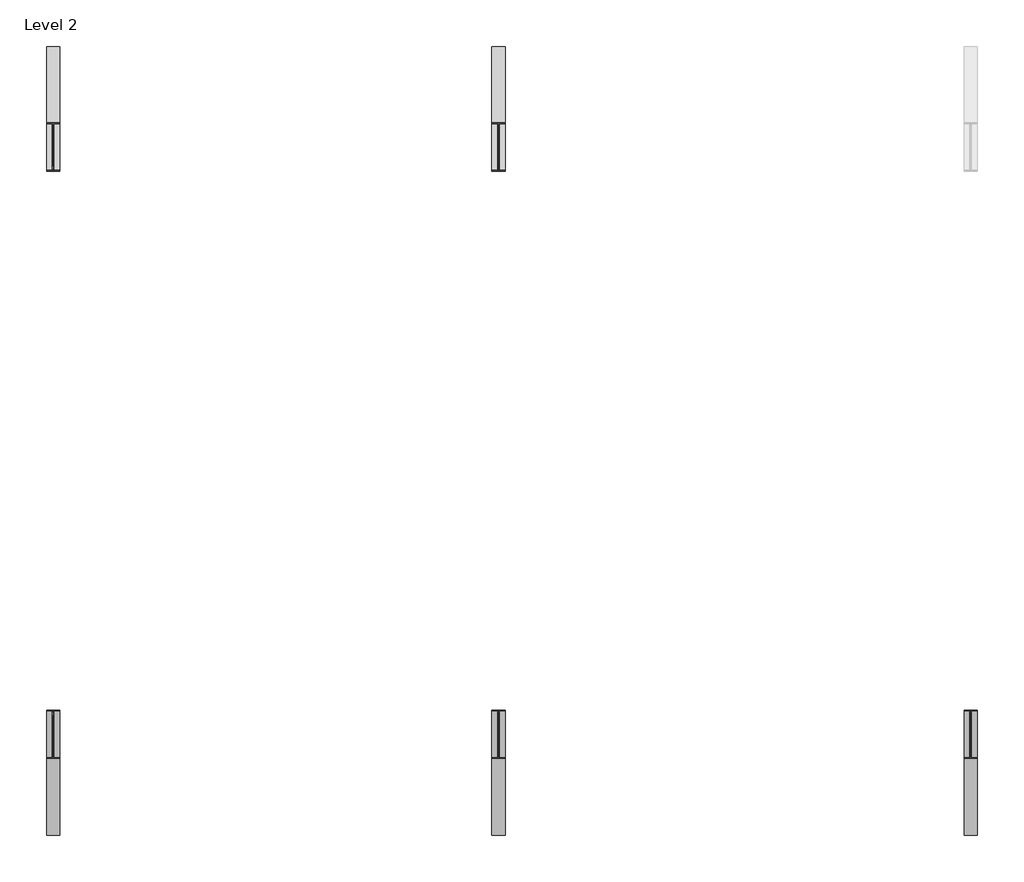
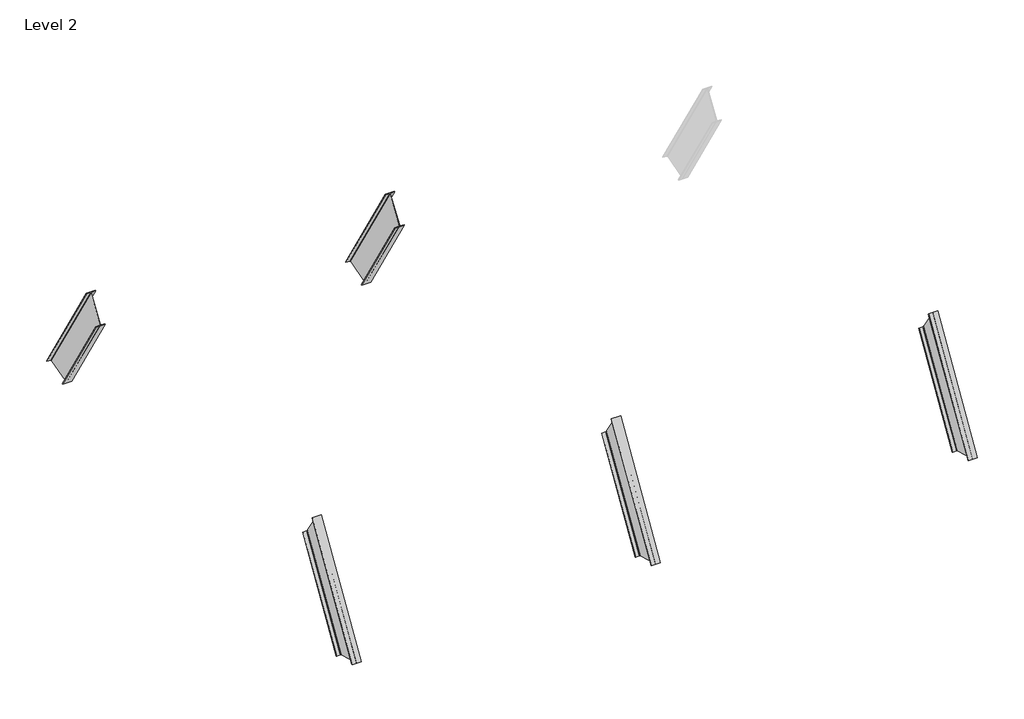
# One storey, part 1 of 2: 5 beams.
"""IFC4 building model written with IfcOpenShell, lengths in millimetres."""

from ifc_helpers import new_model, si_unit, frame, origin, place, context, project, spatial, polyline, ellipse_curve, element, save
from ifc_brep_helpers import plane_surface, revolved_surface, advanced_brep

model = new_model("IFC4")

# Units and contexts
model_context = context("Model", 3, world=origin())
ifc_project = project(units=[si_unit("LENGTHUNIT", "METRE", prefix="MILLI")], contexts=[model_context])

# Site, building, storey
site = spatial("IfcSite", under=ifc_project)
building = spatial("IfcBuilding", under=site)
storey = spatial("IfcBuildingStorey", under=building, Name="Level 2", Elevation=3048.0)

# Beams
placement = place(None, origin())
element("IfcBeam", 1, ObjectType="W Shapes : W 6X18.5", at=placement, inside=storey, context=model_context, shape_type="AdvancedBrep", body=[
    advanced_brep(
    [(18053.8370052, 4087.4629396, 4314.3781499), (17988.1780052, 4087.4629396, 4314.3781499), (17988.1780052, 3103.1094714, 2696.9143292), (18053.8370052, 3103.1094714, 2696.9143292), (17980.5580052, 4082.8387117, 4321.4371423), (17980.5580052, 3095.4894199, 2699.0506628), (17980.5580052, 3818.6411587, 4724.7409096), (17980.5580052, 2660.1304783, 2821.106522), (17988.1780052, 3814.0169308, 4731.799902), (17988.1780052, 2652.5104268, 2823.2428556), (18053.8370052, 3814.0169308, 4731.799902), (18053.8370052, 2652.5104268, 2823.2428556), (18053.8370052, 3808.1595755, 4740.7412924), (18053.8370052, 2642.8583616, 2825.9488782), (17901.4370052, 3808.1595755, 4740.7412924), (17901.4370052, 2642.8583616, 2825.9488782), (17901.4370052, 3814.0169308, 4731.799902), (17901.4370052, 2652.5104268, 2823.2428556), (17967.0960052, 3814.0169308, 4731.799902), (17967.0960052, 2652.5104268, 2823.2428556), (17974.7160052, 3818.6411587, 4724.7409096), (17974.7160052, 2660.1304783, 2821.106522), (17974.7160052, 4082.8387117, 4321.4371423), (17974.7160052, 3095.4894199, 2699.0506628), (17967.0960052, 4087.4629396, 4314.3781499), (17967.0960052, 3103.1094714, 2696.9143292), (17901.4370052, 4087.4629396, 4314.3781499), (17901.4370052, 3103.1094714, 2696.9143292), (17901.4370052, 4093.3202949, 4305.4367595), (17901.4370052, 3112.7615366, 2694.2083066), (18053.8370052, 4093.3202949, 4305.4367595), (18053.8370052, 3112.7615366, 2694.2083066)],
    [
        (0, 1),
        (1, 2),
        (2, 3),
        (3, 0),
        (1, 4, ellipse_curve(frame((17988.1780052, 4082.8387117, 4321.4371423), z_axis=(0.0, 0.8364953080573764, 0.5479740866117624), x_axis=(0.0, 0.5479740866117631, -0.8364953080573758)), 8.4387711, 7.62)),
        (4, 5),
        (5, 2, ellipse_curve(frame((17988.1780052, 3095.4894199, 2699.0506628), z_axis=(0.0, -0.26994852802482067, -0.9628747541696338), x_axis=(0.0, -0.9628747541696336, 0.26994852802482094)), 7.9138553, 7.62)),
        (4, 6),
        (6, 7),
        (7, 5),
        (6, 8, ellipse_curve(frame((17988.1780052, 3818.6411587, 4724.7409096), z_axis=(0.0, 0.8364953080573764, 0.5479740866117624), x_axis=(0.0, 0.5479740866117631, -0.8364953080573758)), 8.4387711, 7.62)),
        (8, 9),
        (9, 7, ellipse_curve(frame((17988.1780052, 2660.1304783, 2821.106522), z_axis=(0.0, -0.26994852802482067, -0.9628747541696338), x_axis=(0.0, -0.9628747541696336, 0.26994852802482094)), 7.9138553, 7.62)),
        (8, 10),
        (10, 11),
        (11, 9),
        (10, 12),
        (12, 13),
        (13, 11),
        (12, 14),
        (14, 15),
        (15, 13),
        (14, 16),
        (16, 17),
        (17, 15),
        (16, 18),
        (18, 19),
        (19, 17),
        (18, 20, ellipse_curve(frame((17967.0960052, 3818.6411587, 4724.7409096), z_axis=(0.0, 0.8364953080573764, 0.5479740866117624), x_axis=(0.0, 0.5479740866117631, -0.8364953080573758)), 8.4387711, 7.62)),
        (20, 21),
        (21, 19, ellipse_curve(frame((17967.0960052, 2660.1304783, 2821.106522), z_axis=(0.0, -0.26994852802482067, -0.9628747541696338), x_axis=(0.0, -0.9628747541696336, 0.26994852802482094)), 7.9138553, 7.62)),
        (20, 22),
        (22, 23),
        (23, 21),
        (22, 24, ellipse_curve(frame((17967.0960052, 4082.8387117, 4321.4371423), z_axis=(0.0, 0.8364953080573764, 0.5479740866117624), x_axis=(0.0, 0.5479740866117631, -0.8364953080573758)), 8.4387711, 7.62)),
        (24, 25),
        (25, 23, ellipse_curve(frame((17967.0960052, 3095.4894199, 2699.0506628), z_axis=(0.0, -0.26994852802482067, -0.9628747541696338), x_axis=(0.0, -0.9628747541696336, 0.26994852802482094)), 7.9138553, 7.62)),
        (24, 26),
        (26, 27),
        (27, 25),
        (26, 28),
        (28, 29),
        (29, 27),
        (28, 30),
        (30, 31),
        (31, 29),
        (30, 0),
        (3, 31),
    ],
    [
        plane_surface(frame((18053.8370052, 4201.324019, 4501.4716915), z_axis=(0.0, -0.8542430559708922, 0.5198738321222864), x_axis=(0.0, -0.5198738321222864, -0.8542430559708922))),
        revolved_surface(polyline([(17980.5580052, 3094.3787005304976, 2697.225557775975), (17980.5580052, 4084.7238158871687, 4324.534696138475)]), (17988.1780052, 4194.8146869, 4505.4331301), (0.0, -0.5198738321222864, -0.8542430559708922)),
        plane_surface(frame((17980.5580052, 4194.8146869, 4505.4331301), z_axis=(1.0000000000000002, 0.0, 0.0), x_axis=(0.0, -0.5198738321222864, -0.8542430559708922))),
        revolved_surface(polyline([(17980.5580052, 2659.0197588679885, 2819.2814170104925), (17980.5580052, 3820.5262629103145, 4727.8384634243885)]), (17988.1780052, 3822.914847, 4731.7633222), (0.0, -0.5198738321222864, -0.8542430559708922)),
        plane_surface(frame((17988.1780052, 3816.405515, 4735.7247608), z_axis=(0.0, 0.8542430559708922, -0.5198738321222864), x_axis=(0.0, -0.5198738321222864, -0.8542430559708922))),
        plane_surface(frame((18053.8370052, 3816.405515, 4735.7247608), z_axis=(1.0000000000000002, 0.0, 0.0), x_axis=(0.0, -0.5198738321222864, -0.8542430559708922))),
        plane_surface(frame((18053.8370052, 3808.160361, 4740.742583), z_axis=(0.0, -0.8542430559708922, 0.5198738321222864), x_axis=(0.0, -0.5198738321222864, -0.8542430559708922))),
        plane_surface(frame((17901.4370052, 3808.160361, 4740.742583), z_axis=(-1.0000000000000002, 0.0, 0.0), x_axis=(0.0, -0.5198738321222864, -0.8542430559708922))),
        plane_surface(frame((17901.4370052, 3816.405515, 4735.7247608), z_axis=(0.0, 0.8542430559708922, -0.5198738321222864), x_axis=(0.0, -0.5198738321222864, -0.8542430559708922))),
        revolved_surface(polyline([(17959.476005200002, 2659.0197588679885, 2819.2814170104925), (17959.476005200002, 3820.5262629103145, 4727.8384634243885)]), (17967.0960052, 3822.914847, 4731.7633222), (0.0, -0.5198738321222864, -0.8542430559708922)),
        plane_surface(frame((17974.7160052, 3822.914847, 4731.7633222), z_axis=(-1.0000000000000002, 0.0, 0.0), x_axis=(0.0, -0.5198738321222864, -0.8542430559708922))),
        revolved_surface(polyline([(17959.476005200002, 3094.3787005304976, 2697.225557775975), (17959.476005200002, 4084.7238158871687, 4324.534696138475)]), (17967.0960052, 4194.8146869, 4505.4331301), (0.0, -0.5198738321222864, -0.8542430559708922)),
        plane_surface(frame((17967.0960052, 4201.324019, 4501.4716915), z_axis=(0.0, -0.8542430559708922, 0.5198738321222864), x_axis=(0.0, -0.5198738321222864, -0.8542430559708922))),
        plane_surface(frame((17901.4370052, 4201.324019, 4501.4716915), z_axis=(-1.0000000000000002, 0.0, 0.0), x_axis=(0.0, -0.5198738321222864, -0.8542430559708922))),
        plane_surface(frame((17901.4370052, 4209.569173, 4496.4538693), z_axis=(0.0, 0.8542430559708922, -0.5198738321222864), x_axis=(0.0, -0.5198738321222864, -0.8542430559708922))),
        plane_surface(frame((18053.8370052, 4209.569173, 4496.4538693), z_axis=(1.0000000000000002, 0.0, 0.0), x_axis=(0.0, -0.5198738321222864, -0.8542430559708922))),
        plane_surface(frame((15602.0985648, 2512.1527504, 2862.5930909), z_axis=(0.0, -0.26994852802482067, -0.9628747541696338), x_axis=(1.0, 0.0, 0.0))),
        plane_surface(frame((17977.6405771, 4093.3183681, 4305.4397008), z_axis=(0.0, 0.8364953080573764, 0.5479740866117624), x_axis=(1.0, 0.0, 0.0))),
    ],
    [
        (0, [[1, 2, 3, 4]]),
        (1, [[5, 6, 7, -2]]),
        (2, [[8, 9, 10, -6]]),
        (3, [[11, 12, 13, -9]]),
        (4, [[14, 15, 16, -12]]),
        (5, [[17, 18, 19, -15]]),
        (6, [[20, 21, 22, -18]]),
        (7, [[23, 24, 25, -21]]),
        (8, [[26, 27, 28, -24]]),
        (9, [[29, 30, 31, -27]]),
        (10, [[32, 33, 34, -30]]),
        (11, [[35, 36, 37, -33]]),
        (12, [[38, 39, 40, -36]]),
        (13, [[41, 42, 43, -39]]),
        (14, [[44, 45, 46, -42]]),
        (15, [[47, -4, 48, -45]]),
        (16, [[-3, -7, -10, -13, -16, -19, -22, -25, -28, -31, -34, -37, -40, -43, -46, -48]]),
        (17, [[-1, -47, -44, -41, -38, -35, -32, -29, -26, -23, -20, -17, -14, -11, -8, -5]]),
    ],
),
])
element("IfcBeam", 2, ObjectType="W Shapes : W 6X18.5", at=placement, inside=storey, context=model_context, shape_type="AdvancedBrep", body=[
    advanced_brep(
    [(12635.1280052, 10139.0601337, 4314.3781499), (12700.7870052, 10139.0601337, 4314.3781499), (12700.7870052, 11123.4136018, 2696.9143292), (12635.1280052, 11123.4136018, 2696.9143292), (12627.5080052, 10143.6843616, 4321.4371423), (12627.5080052, 11131.0336533, 2699.0506628), (12627.5080052, 10407.8819145, 4724.7409096), (12627.5080052, 11566.3925949, 2821.106522), (12635.1280052, 10412.5061424, 4731.799902), (12635.1280052, 11574.0126464, 2823.2428556), (12700.7870052, 10412.5061424, 4731.799902), (12700.7870052, 11574.0126464, 2823.2428556), (12700.7870052, 10418.3634977, 4740.7412924), (12700.7870052, 11583.6647116, 2825.9488782), (12548.3870052, 10418.3634977, 4740.7412924), (12548.3870052, 11583.6647116, 2825.9488782), (12548.3870052, 10412.5061424, 4731.799902), (12548.3870052, 11574.0126464, 2823.2428556), (12614.0460052, 10412.5061424, 4731.799902), (12614.0460052, 11574.0126464, 2823.2428556), (12621.6660052, 10407.8819145, 4724.7409096), (12621.6660052, 11566.3925949, 2821.106522), (12621.6660052, 10143.6843616, 4321.4371423), (12621.6660052, 11131.0336533, 2699.0506628), (12614.0460052, 10139.0601337, 4314.3781499), (12614.0460052, 11123.4136018, 2696.9143292), (12548.3870052, 10139.0601337, 4314.3781499), (12548.3870052, 11123.4136018, 2696.9143292), (12548.3870052, 10133.2027784, 4305.4367595), (12548.3870052, 11113.7615366, 2694.2083066), (12700.7870052, 10133.2027784, 4305.4367595), (12700.7870052, 11113.7615366, 2694.2083066)],
    [
        (0, 1),
        (1, 2),
        (2, 3),
        (3, 0),
        (4, 0, ellipse_curve(frame((12635.1280052, 10143.6843616, 4321.4371423), z_axis=(0.0, -0.836495308057375, 0.5479740866117643), x_axis=(0.0, -0.5479740866117645, -0.8364953080573748)), 8.4387711, 7.62)),
        (3, 5, ellipse_curve(frame((12635.1280052, 11131.0336533, 2699.0506628), z_axis=(0.0, 0.2699485280248213, -0.9628747541696336), x_axis=(0.0, 0.9628747541696333, 0.26994852802482194)), 7.9138553, 7.62)),
        (5, 4),
        (6, 4),
        (5, 7),
        (7, 6),
        (8, 6, ellipse_curve(frame((12635.1280052, 10407.8819145, 4724.7409096), z_axis=(0.0, -0.836495308057375, 0.5479740866117643), x_axis=(0.0, -0.5479740866117645, -0.8364953080573748)), 8.4387711, 7.62)),
        (7, 9, ellipse_curve(frame((12635.1280052, 11566.3925949, 2821.106522), z_axis=(0.0, 0.2699485280248213, -0.9628747541696336), x_axis=(0.0, 0.9628747541696333, 0.26994852802482194)), 7.9138553, 7.62)),
        (9, 8),
        (10, 8),
        (9, 11),
        (11, 10),
        (12, 10),
        (11, 13),
        (13, 12),
        (14, 12),
        (13, 15),
        (15, 14),
        (16, 14),
        (15, 17),
        (17, 16),
        (18, 16),
        (17, 19),
        (19, 18),
        (20, 18, ellipse_curve(frame((12614.0460052, 10407.8819145, 4724.7409096), z_axis=(0.0, -0.836495308057375, 0.5479740866117643), x_axis=(0.0, -0.5479740866117645, -0.8364953080573748)), 8.4387711, 7.62)),
        (19, 21, ellipse_curve(frame((12614.0460052, 11566.3925949, 2821.106522), z_axis=(0.0, 0.2699485280248213, -0.9628747541696336), x_axis=(0.0, 0.9628747541696333, 0.26994852802482194)), 7.9138553, 7.62)),
        (21, 20),
        (22, 20),
        (21, 23),
        (23, 22),
        (24, 22, ellipse_curve(frame((12614.0460052, 10143.6843616, 4321.4371423), z_axis=(0.0, -0.836495308057375, 0.5479740866117643), x_axis=(0.0, -0.5479740866117645, -0.8364953080573748)), 8.4387711, 7.62)),
        (23, 25, ellipse_curve(frame((12614.0460052, 11131.0336533, 2699.0506628), z_axis=(0.0, 0.2699485280248213, -0.9628747541696336), x_axis=(0.0, 0.9628747541696333, 0.26994852802482194)), 7.9138553, 7.62)),
        (25, 24),
        (26, 24),
        (25, 27),
        (27, 26),
        (28, 26),
        (27, 29),
        (29, 28),
        (30, 28),
        (29, 31),
        (31, 30),
        (1, 30),
        (31, 2),
    ],
    [
        plane_surface(frame((12700.7870052, 10025.1990543, 4501.4716915), z_axis=(0.0, 0.8542430559708922, 0.5198738321222864), x_axis=(0.0, 0.5198738321222864, -0.8542430559708922))),
        revolved_surface(polyline([(12627.5080052, 11132.144372669503, 2697.225557775976), (12627.5080052, 10141.799257339859, 4324.534696094065)]), (12635.1280052, 10031.7083863, 4505.4331301), (0.0, 0.5198738321222863, -0.8542430559708921)),
        plane_surface(frame((12627.5080052, 10031.7083863, 4505.4331301), z_axis=(1.0000000000000002, 0.0, 0.0), x_axis=(0.0, 0.5198738321222864, -0.8542430559708922))),
        revolved_surface(polyline([(12627.5080052, 11567.50331433201, 2819.281417010493), (12627.5080052, 10405.996810289686, 4727.8384634243885)]), (12635.1280052, 10403.6082262, 4731.7633222), (0.0, 0.5198738321222863, -0.8542430559708921)),
        plane_surface(frame((12635.1280052, 10410.1175583, 4735.7247608), z_axis=(0.0, -0.8542430559708922, -0.5198738321222864), x_axis=(0.0, 0.5198738321222864, -0.8542430559708922))),
        plane_surface(frame((12700.7870052, 10410.1175583, 4735.7247608), z_axis=(1.0000000000000002, 0.0, 0.0), x_axis=(0.0, 0.5198738321222864, -0.8542430559708922))),
        plane_surface(frame((12700.7870052, 10418.3627123, 4740.742583), z_axis=(0.0, 0.8542430559708922, 0.5198738321222864), x_axis=(0.0, 0.5198738321222864, -0.8542430559708922))),
        plane_surface(frame((12548.3870052, 10418.3627123, 4740.742583), z_axis=(-1.0000000000000002, 0.0, 0.0), x_axis=(0.0, 0.5198738321222864, -0.8542430559708922))),
        plane_surface(frame((12548.3870052, 10410.1175583, 4735.7247608), z_axis=(0.0, -0.8542430559708922, -0.5198738321222864), x_axis=(0.0, 0.5198738321222864, -0.8542430559708922))),
        revolved_surface(polyline([(12606.426005199999, 11567.50331433201, 2819.281417010493), (12606.426005199999, 10405.996810289686, 4727.8384634243885)]), (12614.0460052, 10403.6082262, 4731.7633222), (0.0, 0.5198738321222863, -0.8542430559708921)),
        plane_surface(frame((12621.6660052, 10403.6082262, 4731.7633222), z_axis=(-1.0000000000000002, 0.0, 0.0), x_axis=(0.0, 0.5198738321222864, -0.8542430559708922))),
        revolved_surface(polyline([(12606.426005199999, 11132.144372669503, 2697.225557775976), (12606.426005199999, 10141.799257339859, 4324.534696094065)]), (12614.0460052, 10031.7083863, 4505.4331301), (0.0, 0.5198738321222863, -0.8542430559708921)),
        plane_surface(frame((12614.0460052, 10025.1990543, 4501.4716915), z_axis=(0.0, 0.8542430559708922, 0.5198738321222864), x_axis=(0.0, 0.5198738321222864, -0.8542430559708922))),
        plane_surface(frame((12548.3870052, 10025.1990543, 4501.4716915), z_axis=(-1.0000000000000002, 0.0, 0.0), x_axis=(0.0, 0.5198738321222864, -0.8542430559708922))),
        plane_surface(frame((12548.3870052, 10016.9539003, 4496.4538693), z_axis=(0.0, -0.8542430559708922, -0.5198738321222864), x_axis=(0.0, 0.5198738321222864, -0.8542430559708922))),
        plane_surface(frame((12700.7870052, 10016.9539003, 4496.4538693), z_axis=(1.0000000000000002, 0.0, 0.0), x_axis=(0.0, 0.5198738321222864, -0.8542430559708922))),
        plane_surface(frame((15000.1254456, 11714.3703228, 2862.5930909), z_axis=(0.0, 0.2699485280248213, -0.9628747541696336), x_axis=(-1.0, 0.0, 0.0))),
        plane_surface(frame((12624.5905771, 10418.3654245, 4740.7442336), z_axis=(0.0, -0.836495308057375, 0.5479740866117643), x_axis=(1.0, 0.0, 0.0))),
    ],
    [
        (0, [[1, 2, 3, 4]]),
        (1, [[5, -4, 6, 7]]),
        (2, [[8, -7, 9, 10]]),
        (3, [[11, -10, 12, 13]]),
        (4, [[14, -13, 15, 16]]),
        (5, [[17, -16, 18, 19]]),
        (6, [[20, -19, 21, 22]]),
        (7, [[23, -22, 24, 25]]),
        (8, [[26, -25, 27, 28]]),
        (9, [[29, -28, 30, 31]]),
        (10, [[32, -31, 33, 34]]),
        (11, [[35, -34, 36, 37]]),
        (12, [[38, -37, 39, 40]]),
        (13, [[41, -40, 42, 43]]),
        (14, [[44, -43, 45, 46]]),
        (15, [[47, -46, 48, -2]]),
        (16, [[-3, -48, -45, -42, -39, -36, -33, -30, -27, -24, -21, -18, -15, -12, -9, -6]]),
        (17, [[-1, -5, -8, -11, -14, -17, -20, -23, -26, -29, -32, -35, -38, -41, -44, -47]]),
    ],
),
])
element("IfcBeam", 3, ObjectType="W Shapes : W 6X18.5", at=placement, inside=storey, context=model_context, shape_type="AdvancedBrep", body=[
    advanced_brep(
    [(12700.7870052, 4087.4629396, 4314.3781499), (12635.1280052, 4087.4629396, 4314.3781499), (12635.1280052, 3103.1094714, 2696.9143292), (12700.7870052, 3103.1094714, 2696.9143292), (12627.5080052, 4082.8387117, 4321.4371423), (12627.5080052, 3095.4894199, 2699.0506628), (12627.5080052, 3818.6411587, 4724.7409096), (12627.5080052, 2660.1304783, 2821.106522), (12635.1280052, 3814.0169308, 4731.799902), (12635.1280052, 2652.5104268, 2823.2428556), (12700.7870052, 3814.0169308, 4731.799902), (12700.7870052, 2652.5104268, 2823.2428556), (12700.7870052, 3808.1595755, 4740.7412924), (12700.7870052, 2642.8583616, 2825.9488782), (12548.3870052, 3808.1595755, 4740.7412924), (12548.3870052, 2642.8583616, 2825.9488782), (12548.3870052, 3814.0169308, 4731.799902), (12548.3870052, 2652.5104268, 2823.2428556), (12614.0460052, 3814.0169308, 4731.799902), (12614.0460052, 2652.5104268, 2823.2428556), (12621.6660052, 3818.6411587, 4724.7409096), (12621.6660052, 2660.1304783, 2821.106522), (12621.6660052, 4082.8387117, 4321.4371423), (12621.6660052, 3095.4894199, 2699.0506628), (12614.0460052, 4087.4629396, 4314.3781499), (12614.0460052, 3103.1094714, 2696.9143292), (12548.3870052, 4087.4629396, 4314.3781499), (12548.3870052, 3103.1094714, 2696.9143292), (12548.3870052, 4093.3202949, 4305.4367595), (12548.3870052, 3112.7615366, 2694.2083066), (12700.7870052, 4093.3202949, 4305.4367595), (12700.7870052, 3112.7615366, 2694.2083066)],
    [
        (0, 1),
        (1, 2),
        (2, 3),
        (3, 0),
        (1, 4, ellipse_curve(frame((12635.1280052, 4082.8387117, 4321.4371423), z_axis=(0.0, 0.8364953080573764, 0.5479740866117624), x_axis=(0.0, 0.5479740866117631, -0.8364953080573758)), 8.4387711, 7.62)),
        (4, 5),
        (5, 2, ellipse_curve(frame((12635.1280052, 3095.4894199, 2699.0506628), z_axis=(0.0, -0.26994852802482067, -0.9628747541696338), x_axis=(0.0, -0.9628747541696336, 0.26994852802482094)), 7.9138553, 7.62)),
        (4, 6),
        (6, 7),
        (7, 5),
        (6, 8, ellipse_curve(frame((12635.1280052, 3818.6411587, 4724.7409096), z_axis=(0.0, 0.8364953080573764, 0.5479740866117624), x_axis=(0.0, 0.5479740866117631, -0.8364953080573758)), 8.4387711, 7.62)),
        (8, 9),
        (9, 7, ellipse_curve(frame((12635.1280052, 2660.1304783, 2821.106522), z_axis=(0.0, -0.26994852802482067, -0.9628747541696338), x_axis=(0.0, -0.9628747541696336, 0.26994852802482094)), 7.9138553, 7.62)),
        (8, 10),
        (10, 11),
        (11, 9),
        (10, 12),
        (12, 13),
        (13, 11),
        (12, 14),
        (14, 15),
        (15, 13),
        (14, 16),
        (16, 17),
        (17, 15),
        (16, 18),
        (18, 19),
        (19, 17),
        (18, 20, ellipse_curve(frame((12614.0460052, 3818.6411587, 4724.7409096), z_axis=(0.0, 0.8364953080573764, 0.5479740866117624), x_axis=(0.0, 0.5479740866117631, -0.8364953080573758)), 8.4387711, 7.62)),
        (20, 21),
        (21, 19, ellipse_curve(frame((12614.0460052, 2660.1304783, 2821.106522), z_axis=(0.0, -0.26994852802482067, -0.9628747541696338), x_axis=(0.0, -0.9628747541696336, 0.26994852802482094)), 7.9138553, 7.62)),
        (20, 22),
        (22, 23),
        (23, 21),
        (22, 24, ellipse_curve(frame((12614.0460052, 4082.8387117, 4321.4371423), z_axis=(0.0, 0.8364953080573764, 0.5479740866117624), x_axis=(0.0, 0.5479740866117631, -0.8364953080573758)), 8.4387711, 7.62)),
        (24, 25),
        (25, 23, ellipse_curve(frame((12614.0460052, 3095.4894199, 2699.0506628), z_axis=(0.0, -0.26994852802482067, -0.9628747541696338), x_axis=(0.0, -0.9628747541696336, 0.26994852802482094)), 7.9138553, 7.62)),
        (24, 26),
        (26, 27),
        (27, 25),
        (26, 28),
        (28, 29),
        (29, 27),
        (28, 30),
        (30, 31),
        (31, 29),
        (30, 0),
        (3, 31),
    ],
    [
        plane_surface(frame((12700.7870052, 4201.324019, 4501.4716915), z_axis=(0.0, -0.8542430559708922, 0.5198738321222864), x_axis=(0.0, -0.5198738321222864, -0.8542430559708922))),
        revolved_surface(polyline([(12627.5080052, 3094.3787005304976, 2697.225557775975), (12627.5080052, 4084.7238158871687, 4324.534696138475)]), (12635.1280052, 4194.8146869, 4505.4331301), (0.0, -0.5198738321222864, -0.8542430559708922)),
        plane_surface(frame((12627.5080052, 4194.8146869, 4505.4331301), z_axis=(1.0000000000000002, 0.0, 0.0), x_axis=(0.0, -0.5198738321222864, -0.8542430559708922))),
        revolved_surface(polyline([(12627.5080052, 2659.0197588679885, 2819.2814170104925), (12627.5080052, 3820.5262629103145, 4727.8384634243885)]), (12635.1280052, 3822.914847, 4731.7633222), (0.0, -0.5198738321222864, -0.8542430559708922)),
        plane_surface(frame((12635.1280052, 3816.405515, 4735.7247608), z_axis=(0.0, 0.8542430559708922, -0.5198738321222864), x_axis=(0.0, -0.5198738321222864, -0.8542430559708922))),
        plane_surface(frame((12700.7870052, 3816.405515, 4735.7247608), z_axis=(1.0000000000000002, 0.0, 0.0), x_axis=(0.0, -0.5198738321222864, -0.8542430559708922))),
        plane_surface(frame((12700.7870052, 3808.160361, 4740.742583), z_axis=(0.0, -0.8542430559708922, 0.5198738321222864), x_axis=(0.0, -0.5198738321222864, -0.8542430559708922))),
        plane_surface(frame((12548.3870052, 3808.160361, 4740.742583), z_axis=(-1.0000000000000002, 0.0, 0.0), x_axis=(0.0, -0.5198738321222864, -0.8542430559708922))),
        plane_surface(frame((12548.3870052, 3816.405515, 4735.7247608), z_axis=(0.0, 0.8542430559708922, -0.5198738321222864), x_axis=(0.0, -0.5198738321222864, -0.8542430559708922))),
        revolved_surface(polyline([(12606.426005199999, 2659.0197588679885, 2819.2814170104925), (12606.426005199999, 3820.5262629103145, 4727.8384634243885)]), (12614.0460052, 3822.914847, 4731.7633222), (0.0, -0.5198738321222864, -0.8542430559708922)),
        plane_surface(frame((12621.6660052, 3822.914847, 4731.7633222), z_axis=(-1.0000000000000002, 0.0, 0.0), x_axis=(0.0, -0.5198738321222864, -0.8542430559708922))),
        revolved_surface(polyline([(12606.426005199999, 3094.3787005304976, 2697.225557775975), (12606.426005199999, 4084.7238158871687, 4324.534696138475)]), (12614.0460052, 4194.8146869, 4505.4331301), (0.0, -0.5198738321222864, -0.8542430559708922)),
        plane_surface(frame((12614.0460052, 4201.324019, 4501.4716915), z_axis=(0.0, -0.8542430559708922, 0.5198738321222864), x_axis=(0.0, -0.5198738321222864, -0.8542430559708922))),
        plane_surface(frame((12548.3870052, 4201.324019, 4501.4716915), z_axis=(-1.0000000000000002, 0.0, 0.0), x_axis=(0.0, -0.5198738321222864, -0.8542430559708922))),
        plane_surface(frame((12548.3870052, 4209.569173, 4496.4538693), z_axis=(0.0, 0.8542430559708922, -0.5198738321222864), x_axis=(0.0, -0.5198738321222864, -0.8542430559708922))),
        plane_surface(frame((12700.7870052, 4209.569173, 4496.4538693), z_axis=(1.0000000000000002, 0.0, 0.0), x_axis=(0.0, -0.5198738321222864, -0.8542430559708922))),
        plane_surface(frame((10249.0485648, 2512.1527504, 2862.5930909), z_axis=(0.0, -0.26994852802482067, -0.9628747541696338), x_axis=(1.0, 0.0, 0.0))),
        plane_surface(frame((12624.5905771, 4093.3183681, 4305.4397008), z_axis=(0.0, 0.8364953080573764, 0.5479740866117624), x_axis=(1.0, 0.0, 0.0))),
    ],
    [
        (0, [[1, 2, 3, 4]]),
        (1, [[5, 6, 7, -2]]),
        (2, [[8, 9, 10, -6]]),
        (3, [[11, 12, 13, -9]]),
        (4, [[14, 15, 16, -12]]),
        (5, [[17, 18, 19, -15]]),
        (6, [[20, 21, 22, -18]]),
        (7, [[23, 24, 25, -21]]),
        (8, [[26, 27, 28, -24]]),
        (9, [[29, 30, 31, -27]]),
        (10, [[32, 33, 34, -30]]),
        (11, [[35, 36, 37, -33]]),
        (12, [[38, 39, 40, -36]]),
        (13, [[41, 42, 43, -39]]),
        (14, [[44, 45, 46, -42]]),
        (15, [[47, -4, 48, -45]]),
        (16, [[-3, -7, -10, -13, -16, -19, -22, -25, -28, -31, -34, -37, -40, -43, -46, -48]]),
        (17, [[-1, -47, -44, -41, -38, -35, -32, -29, -26, -23, -20, -17, -14, -11, -8, -5]]),
    ],
),
])
element("IfcBeam", 4, ObjectType="W Shapes : W 6X18.5", at=placement, inside=storey, context=model_context, shape_type="AdvancedBrep", body=[
    advanced_brep(
    [(7586.8780052, 10139.0601337, 4314.3781499), (7652.5370052, 10139.0601337, 4314.3781499), (7652.5370052, 11123.4136018, 2696.9143292), (7586.8780052, 11123.4136018, 2696.9143292), (7579.2580052, 10143.6843616, 4321.4371423), (7579.2580052, 11131.0336533, 2699.0506628), (7579.2580052, 10407.8819145, 4724.7409096), (7579.2580052, 11566.3925949, 2821.106522), (7586.8780052, 10412.5061424, 4731.799902), (7586.8780052, 11574.0126464, 2823.2428556), (7652.5370052, 10412.5061424, 4731.799902), (7652.5370052, 11574.0126464, 2823.2428556), (7652.5370052, 10418.3634977, 4740.7412924), (7652.5370052, 11583.6647116, 2825.9488782), (7500.1370052, 10418.3634977, 4740.7412924), (7500.1370052, 11583.6647116, 2825.9488782), (7500.1370052, 10412.5061424, 4731.799902), (7500.1370052, 11574.0126464, 2823.2428556), (7565.7960052, 10412.5061424, 4731.799902), (7565.7960052, 11574.0126464, 2823.2428556), (7573.4160052, 10407.8819145, 4724.7409096), (7573.4160052, 11566.3925949, 2821.106522), (7573.4160052, 10143.6843616, 4321.4371423), (7573.4160052, 11131.0336533, 2699.0506628), (7565.7960052, 10139.0601337, 4314.3781499), (7565.7960052, 11123.4136018, 2696.9143292), (7500.1370052, 10139.0601337, 4314.3781499), (7500.1370052, 11123.4136018, 2696.9143292), (7500.1370052, 10133.2027784, 4305.4367595), (7500.1370052, 11113.7615366, 2694.2083066), (7652.5370052, 10133.2027784, 4305.4367595), (7652.5370052, 11113.7615366, 2694.2083066)],
    [
        (0, 1),
        (1, 2),
        (2, 3),
        (3, 0),
        (4, 0, ellipse_curve(frame((7586.8780052, 10143.6843616, 4321.4371423), z_axis=(0.0, -0.836495308057375, 0.5479740866117643), x_axis=(0.0, -0.5479740866117645, -0.8364953080573748)), 8.4387711, 7.62)),
        (3, 5, ellipse_curve(frame((7586.8780052, 11131.0336533, 2699.0506628), z_axis=(0.0, 0.2699485280248213, -0.9628747541696336), x_axis=(0.0, 0.9628747541696333, 0.26994852802482194)), 7.9138553, 7.62)),
        (5, 4),
        (6, 4),
        (5, 7),
        (7, 6),
        (8, 6, ellipse_curve(frame((7586.8780052, 10407.8819145, 4724.7409096), z_axis=(0.0, -0.836495308057375, 0.5479740866117643), x_axis=(0.0, -0.5479740866117645, -0.8364953080573748)), 8.4387711, 7.62)),
        (7, 9, ellipse_curve(frame((7586.8780052, 11566.3925949, 2821.106522), z_axis=(0.0, 0.2699485280248213, -0.9628747541696336), x_axis=(0.0, 0.9628747541696333, 0.26994852802482194)), 7.9138553, 7.62)),
        (9, 8),
        (10, 8),
        (9, 11),
        (11, 10),
        (12, 10),
        (11, 13),
        (13, 12),
        (14, 12),
        (13, 15),
        (15, 14),
        (16, 14),
        (15, 17),
        (17, 16),
        (18, 16),
        (17, 19),
        (19, 18),
        (20, 18, ellipse_curve(frame((7565.7960052, 10407.8819145, 4724.7409096), z_axis=(0.0, -0.836495308057375, 0.5479740866117643), x_axis=(0.0, -0.5479740866117645, -0.8364953080573748)), 8.4387711, 7.62)),
        (19, 21, ellipse_curve(frame((7565.7960052, 11566.3925949, 2821.106522), z_axis=(0.0, 0.2699485280248213, -0.9628747541696336), x_axis=(0.0, 0.9628747541696333, 0.26994852802482194)), 7.9138553, 7.62)),
        (21, 20),
        (22, 20),
        (21, 23),
        (23, 22),
        (24, 22, ellipse_curve(frame((7565.7960052, 10143.6843616, 4321.4371423), z_axis=(0.0, -0.836495308057375, 0.5479740866117643), x_axis=(0.0, -0.5479740866117645, -0.8364953080573748)), 8.4387711, 7.62)),
        (23, 25, ellipse_curve(frame((7565.7960052, 11131.0336533, 2699.0506628), z_axis=(0.0, 0.2699485280248213, -0.9628747541696336), x_axis=(0.0, 0.9628747541696333, 0.26994852802482194)), 7.9138553, 7.62)),
        (25, 24),
        (26, 24),
        (25, 27),
        (27, 26),
        (28, 26),
        (27, 29),
        (29, 28),
        (30, 28),
        (29, 31),
        (31, 30),
        (1, 30),
        (31, 2),
    ],
    [
        plane_surface(frame((7652.5370052, 10025.1990543, 4501.4716915), z_axis=(0.0, 0.8542430559708922, 0.5198738321222864), x_axis=(0.0, 0.5198738321222864, -0.8542430559708922))),
        revolved_surface(polyline([(7579.2580052, 11132.144372669503, 2697.225557775976), (7579.2580052, 10141.799257339859, 4324.534696094065)]), (7586.8780052, 10031.7083863, 4505.4331301), (0.0, 0.5198738321222863, -0.8542430559708921)),
        plane_surface(frame((7579.2580052, 10031.7083863, 4505.4331301), z_axis=(1.0000000000000002, 0.0, 0.0), x_axis=(0.0, 0.5198738321222864, -0.8542430559708922))),
        revolved_surface(polyline([(7579.2580052, 11567.50331433201, 2819.281417010493), (7579.2580052, 10405.996810289686, 4727.8384634243885)]), (7586.8780052, 10403.6082262, 4731.7633222), (0.0, 0.5198738321222863, -0.8542430559708921)),
        plane_surface(frame((7586.8780052, 10410.1175583, 4735.7247608), z_axis=(0.0, -0.8542430559708922, -0.5198738321222864), x_axis=(0.0, 0.5198738321222864, -0.8542430559708922))),
        plane_surface(frame((7652.5370052, 10410.1175583, 4735.7247608), z_axis=(1.0000000000000002, 0.0, 0.0), x_axis=(0.0, 0.5198738321222864, -0.8542430559708922))),
        plane_surface(frame((7652.5370052, 10418.3627123, 4740.742583), z_axis=(0.0, 0.8542430559708922, 0.5198738321222864), x_axis=(0.0, 0.5198738321222864, -0.8542430559708922))),
        plane_surface(frame((7500.1370052, 10418.3627123, 4740.742583), z_axis=(-1.0000000000000002, 0.0, 0.0), x_axis=(0.0, 0.5198738321222864, -0.8542430559708922))),
        plane_surface(frame((7500.1370052, 10410.1175583, 4735.7247608), z_axis=(0.0, -0.8542430559708922, -0.5198738321222864), x_axis=(0.0, 0.5198738321222864, -0.8542430559708922))),
        revolved_surface(polyline([(7558.1760052, 11567.50331433201, 2819.281417010493), (7558.1760052, 10405.996810289686, 4727.8384634243885)]), (7565.7960052, 10403.6082262, 4731.7633222), (0.0, 0.5198738321222863, -0.8542430559708921)),
        plane_surface(frame((7573.4160052, 10403.6082262, 4731.7633222), z_axis=(-1.0000000000000002, 0.0, 0.0), x_axis=(0.0, 0.5198738321222864, -0.8542430559708922))),
        revolved_surface(polyline([(7558.1760052, 11132.144372669503, 2697.225557775976), (7558.1760052, 10141.799257339859, 4324.534696094065)]), (7565.7960052, 10031.7083863, 4505.4331301), (0.0, 0.5198738321222863, -0.8542430559708921)),
        plane_surface(frame((7565.7960052, 10025.1990543, 4501.4716915), z_axis=(0.0, 0.8542430559708922, 0.5198738321222864), x_axis=(0.0, 0.5198738321222864, -0.8542430559708922))),
        plane_surface(frame((7500.1370052, 10025.1990543, 4501.4716915), z_axis=(-1.0000000000000002, 0.0, 0.0), x_axis=(0.0, 0.5198738321222864, -0.8542430559708922))),
        plane_surface(frame((7500.1370052, 10016.9539003, 4496.4538693), z_axis=(0.0, -0.8542430559708922, -0.5198738321222864), x_axis=(0.0, 0.5198738321222864, -0.8542430559708922))),
        plane_surface(frame((7652.5370052, 10016.9539003, 4496.4538693), z_axis=(1.0000000000000002, 0.0, 0.0), x_axis=(0.0, 0.5198738321222864, -0.8542430559708922))),
        plane_surface(frame((9951.8754456, 11714.3703228, 2862.5930909), z_axis=(0.0, 0.2699485280248213, -0.9628747541696336), x_axis=(-1.0, 0.0, 0.0))),
        plane_surface(frame((7576.3405771, 10418.3654245, 4740.7442336), z_axis=(0.0, -0.836495308057375, 0.5479740866117643), x_axis=(1.0, 0.0, 0.0))),
    ],
    [
        (0, [[1, 2, 3, 4]]),
        (1, [[5, -4, 6, 7]]),
        (2, [[8, -7, 9, 10]]),
        (3, [[11, -10, 12, 13]]),
        (4, [[14, -13, 15, 16]]),
        (5, [[17, -16, 18, 19]]),
        (6, [[20, -19, 21, 22]]),
        (7, [[23, -22, 24, 25]]),
        (8, [[26, -25, 27, 28]]),
        (9, [[29, -28, 30, 31]]),
        (10, [[32, -31, 33, 34]]),
        (11, [[35, -34, 36, 37]]),
        (12, [[38, -37, 39, 40]]),
        (13, [[41, -40, 42, 43]]),
        (14, [[44, -43, 45, 46]]),
        (15, [[47, -46, 48, -2]]),
        (16, [[-3, -48, -45, -42, -39, -36, -33, -30, -27, -24, -21, -18, -15, -12, -9, -6]]),
        (17, [[-1, -5, -8, -11, -14, -17, -20, -23, -26, -29, -32, -35, -38, -41, -44, -47]]),
    ],
),
])
element("IfcBeam", 5, ObjectType="W Shapes : W 6X18.5", at=placement, inside=storey, context=model_context, shape_type="AdvancedBrep", body=[
    advanced_brep(
    [(7652.5370052, 4087.4629396, 4314.3781499), (7586.8780052, 4087.4629396, 4314.3781499), (7586.8780052, 3103.1094714, 2696.9143292), (7652.5370052, 3103.1094714, 2696.9143292), (7579.2580052, 4082.8387117, 4321.4371423), (7579.2580052, 3095.4894199, 2699.0506628), (7579.2580052, 3818.6411587, 4724.7409096), (7579.2580052, 2660.1304783, 2821.106522), (7586.8780052, 3814.0169308, 4731.799902), (7586.8780052, 2652.5104268, 2823.2428556), (7652.5370052, 3814.0169308, 4731.799902), (7652.5370052, 2652.5104268, 2823.2428556), (7652.5370052, 3808.1595755, 4740.7412924), (7652.5370052, 2642.8583616, 2825.9488782), (7500.1370052, 3808.1595755, 4740.7412924), (7500.1370052, 2642.8583616, 2825.9488782), (7500.1370052, 3814.0169308, 4731.799902), (7500.1370052, 2652.5104268, 2823.2428556), (7565.7960052, 3814.0169308, 4731.799902), (7565.7960052, 2652.5104268, 2823.2428556), (7573.4160052, 3818.6411587, 4724.7409096), (7573.4160052, 2660.1304783, 2821.106522), (7573.4160052, 4082.8387117, 4321.4371423), (7573.4160052, 3095.4894199, 2699.0506628), (7565.7960052, 4087.4629396, 4314.3781499), (7565.7960052, 3103.1094714, 2696.9143292), (7500.1370052, 4087.4629396, 4314.3781499), (7500.1370052, 3103.1094714, 2696.9143292), (7500.1370052, 4093.3202949, 4305.4367595), (7500.1370052, 3112.7615366, 2694.2083066), (7652.5370052, 4093.3202949, 4305.4367595), (7652.5370052, 3112.7615366, 2694.2083066)],
    [
        (0, 1),
        (1, 2),
        (2, 3),
        (3, 0),
        (1, 4, ellipse_curve(frame((7586.8780052, 4082.8387117, 4321.4371423), z_axis=(0.0, 0.8364953080573764, 0.5479740866117624), x_axis=(0.0, 0.5479740866117631, -0.8364953080573758)), 8.4387711, 7.62)),
        (4, 5),
        (5, 2, ellipse_curve(frame((7586.8780052, 3095.4894199, 2699.0506628), z_axis=(0.0, -0.26994852802482067, -0.9628747541696338), x_axis=(0.0, -0.9628747541696336, 0.26994852802482094)), 7.9138553, 7.62)),
        (4, 6),
        (6, 7),
        (7, 5),
        (6, 8, ellipse_curve(frame((7586.8780052, 3818.6411587, 4724.7409096), z_axis=(0.0, 0.8364953080573764, 0.5479740866117624), x_axis=(0.0, 0.5479740866117631, -0.8364953080573758)), 8.4387711, 7.62)),
        (8, 9),
        (9, 7, ellipse_curve(frame((7586.8780052, 2660.1304783, 2821.106522), z_axis=(0.0, -0.26994852802482067, -0.9628747541696338), x_axis=(0.0, -0.9628747541696336, 0.26994852802482094)), 7.9138553, 7.62)),
        (8, 10),
        (10, 11),
        (11, 9),
        (10, 12),
        (12, 13),
        (13, 11),
        (12, 14),
        (14, 15),
        (15, 13),
        (14, 16),
        (16, 17),
        (17, 15),
        (16, 18),
        (18, 19),
        (19, 17),
        (18, 20, ellipse_curve(frame((7565.7960052, 3818.6411587, 4724.7409096), z_axis=(0.0, 0.8364953080573764, 0.5479740866117624), x_axis=(0.0, 0.5479740866117631, -0.8364953080573758)), 8.4387711, 7.62)),
        (20, 21),
        (21, 19, ellipse_curve(frame((7565.7960052, 2660.1304783, 2821.106522), z_axis=(0.0, -0.26994852802482067, -0.9628747541696338), x_axis=(0.0, -0.9628747541696336, 0.26994852802482094)), 7.9138553, 7.62)),
        (20, 22),
        (22, 23),
        (23, 21),
        (22, 24, ellipse_curve(frame((7565.7960052, 4082.8387117, 4321.4371423), z_axis=(0.0, 0.8364953080573764, 0.5479740866117624), x_axis=(0.0, 0.5479740866117631, -0.8364953080573758)), 8.4387711, 7.62)),
        (24, 25),
        (25, 23, ellipse_curve(frame((7565.7960052, 3095.4894199, 2699.0506628), z_axis=(0.0, -0.26994852802482067, -0.9628747541696338), x_axis=(0.0, -0.9628747541696336, 0.26994852802482094)), 7.9138553, 7.62)),
        (24, 26),
        (26, 27),
        (27, 25),
        (26, 28),
        (28, 29),
        (29, 27),
        (28, 30),
        (30, 31),
        (31, 29),
        (30, 0),
        (3, 31),
    ],
    [
        plane_surface(frame((7652.5370052, 4201.324019, 4501.4716915), z_axis=(0.0, -0.8542430559708922, 0.5198738321222864), x_axis=(0.0, -0.5198738321222864, -0.8542430559708922))),
        revolved_surface(polyline([(7579.2580052, 3094.3787005304976, 2697.225557775975), (7579.2580052, 4084.7238158871687, 4324.534696138475)]), (7586.8780052, 4194.8146869, 4505.4331301), (0.0, -0.5198738321222864, -0.8542430559708922)),
        plane_surface(frame((7579.2580052, 4194.8146869, 4505.4331301), z_axis=(1.0000000000000002, 0.0, 0.0), x_axis=(0.0, -0.5198738321222864, -0.8542430559708922))),
        revolved_surface(polyline([(7579.2580052, 2659.0197588679885, 2819.2814170104925), (7579.2580052, 3820.5262629103145, 4727.8384634243885)]), (7586.8780052, 3822.914847, 4731.7633222), (0.0, -0.5198738321222864, -0.8542430559708922)),
        plane_surface(frame((7586.8780052, 3816.405515, 4735.7247608), z_axis=(0.0, 0.8542430559708922, -0.5198738321222864), x_axis=(0.0, -0.5198738321222864, -0.8542430559708922))),
        plane_surface(frame((7652.5370052, 3816.405515, 4735.7247608), z_axis=(1.0000000000000002, 0.0, 0.0), x_axis=(0.0, -0.5198738321222864, -0.8542430559708922))),
        plane_surface(frame((7652.5370052, 3808.160361, 4740.742583), z_axis=(0.0, -0.8542430559708922, 0.5198738321222864), x_axis=(0.0, -0.5198738321222864, -0.8542430559708922))),
        plane_surface(frame((7500.1370052, 3808.160361, 4740.742583), z_axis=(-1.0000000000000002, 0.0, 0.0), x_axis=(0.0, -0.5198738321222864, -0.8542430559708922))),
        plane_surface(frame((7500.1370052, 3816.405515, 4735.7247608), z_axis=(0.0, 0.8542430559708922, -0.5198738321222864), x_axis=(0.0, -0.5198738321222864, -0.8542430559708922))),
        revolved_surface(polyline([(7558.1760052, 2659.0197588679885, 2819.2814170104925), (7558.1760052, 3820.5262629103145, 4727.8384634243885)]), (7565.7960052, 3822.914847, 4731.7633222), (0.0, -0.5198738321222864, -0.8542430559708922)),
        plane_surface(frame((7573.4160052, 3822.914847, 4731.7633222), z_axis=(-1.0000000000000002, 0.0, 0.0), x_axis=(0.0, -0.5198738321222864, -0.8542430559708922))),
        revolved_surface(polyline([(7558.1760052, 3094.3787005304976, 2697.225557775975), (7558.1760052, 4084.7238158871687, 4324.534696138475)]), (7565.7960052, 4194.8146869, 4505.4331301), (0.0, -0.5198738321222864, -0.8542430559708922)),
        plane_surface(frame((7565.7960052, 4201.324019, 4501.4716915), z_axis=(0.0, -0.8542430559708922, 0.5198738321222864), x_axis=(0.0, -0.5198738321222864, -0.8542430559708922))),
        plane_surface(frame((7500.1370052, 4201.324019, 4501.4716915), z_axis=(-1.0000000000000002, 0.0, 0.0), x_axis=(0.0, -0.5198738321222864, -0.8542430559708922))),
        plane_surface(frame((7500.1370052, 4209.569173, 4496.4538693), z_axis=(0.0, 0.8542430559708922, -0.5198738321222864), x_axis=(0.0, -0.5198738321222864, -0.8542430559708922))),
        plane_surface(frame((7652.5370052, 4209.569173, 4496.4538693), z_axis=(1.0000000000000002, 0.0, 0.0), x_axis=(0.0, -0.5198738321222864, -0.8542430559708922))),
        plane_surface(frame((5200.7985648, 2512.1527504, 2862.5930909), z_axis=(0.0, -0.26994852802482067, -0.9628747541696338), x_axis=(1.0, 0.0, 0.0))),
        plane_surface(frame((7576.3405771, 4093.3183681, 4305.4397008), z_axis=(0.0, 0.8364953080573764, 0.5479740866117624), x_axis=(1.0, 0.0, 0.0))),
    ],
    [
        (0, [[1, 2, 3, 4]]),
        (1, [[5, 6, 7, -2]]),
        (2, [[8, 9, 10, -6]]),
        (3, [[11, 12, 13, -9]]),
        (4, [[14, 15, 16, -12]]),
        (5, [[17, 18, 19, -15]]),
        (6, [[20, 21, 22, -18]]),
        (7, [[23, 24, 25, -21]]),
        (8, [[26, 27, 28, -24]]),
        (9, [[29, 30, 31, -27]]),
        (10, [[32, 33, 34, -30]]),
        (11, [[35, 36, 37, -33]]),
        (12, [[38, 39, 40, -36]]),
        (13, [[41, 42, 43, -39]]),
        (14, [[44, 45, 46, -42]]),
        (15, [[47, -4, 48, -45]]),
        (16, [[-3, -7, -10, -13, -16, -19, -22, -25, -28, -31, -34, -37, -40, -43, -46, -48]]),
        (17, [[-1, -47, -44, -41, -38, -35, -32, -29, -26, -23, -20, -17, -14, -11, -8, -5]]),
    ],
),
])

save(model, "model.ifc")

# Revit data of these elements
# Type "W Shapes : W 6X18.5"
#   Section Name Key = "W12x26"
#   Assembly Code = "B10"
#   Width = 152.4 mm
#   Web Thickness = 5.842 mm
#   Web Fillet = 7.62 mm
#   Warping Constant = 163001.3 cm⁶
#   Torsional Moment of Inertia = 12.4869 cm⁴
#   Section Area = 7.65 in²
#   Plastic Modulus weak axis = 0.00472801 (stored number, unit not read)
#   Plastic Modulus strong axis = 0.0215278 (stored number, unit not read)
#   Perimeter = 15.0571 m²/m
#   Nominal Weight = 379.441 N/m
#   Moment of Inertia weak axis = 720.08 cm⁴
#   Moment of Inertia strong axis = 8491.12 cm⁴
#   Height = 469.9 mm
#   Flange Thickness = 9.652 mm
#   Elastic Modulus weak axis = 0.00309028 (stored number, unit not read)
#   Elastic Modulus strong axis = 0.0193287 (stored number, unit not read)
#   Centroid Vertical = 234.95 mm
#   Centroid Horizontal = 76.2 mm
#   Length [instance default] = 5' - 0"
#   Structural Material [instance default] = Steel ASTM A992
#   Principal Axes Angle = 0
# Elements 1, 2, 3, 4, 5 (IfcBeam, "W Shapes : W 6X18.5")
#   Comments = ""
#   Structural Material = Steel ASTM A992
#   Phase Created = New Construction
#   Materials on its faces: "Steel ASTM A992"
# Materials
#   "Steel ASTM A992": class "Metal", colour RGB 189 187 185, transparency 0, Description = "Structural steel 50ksi", Cost = 0
